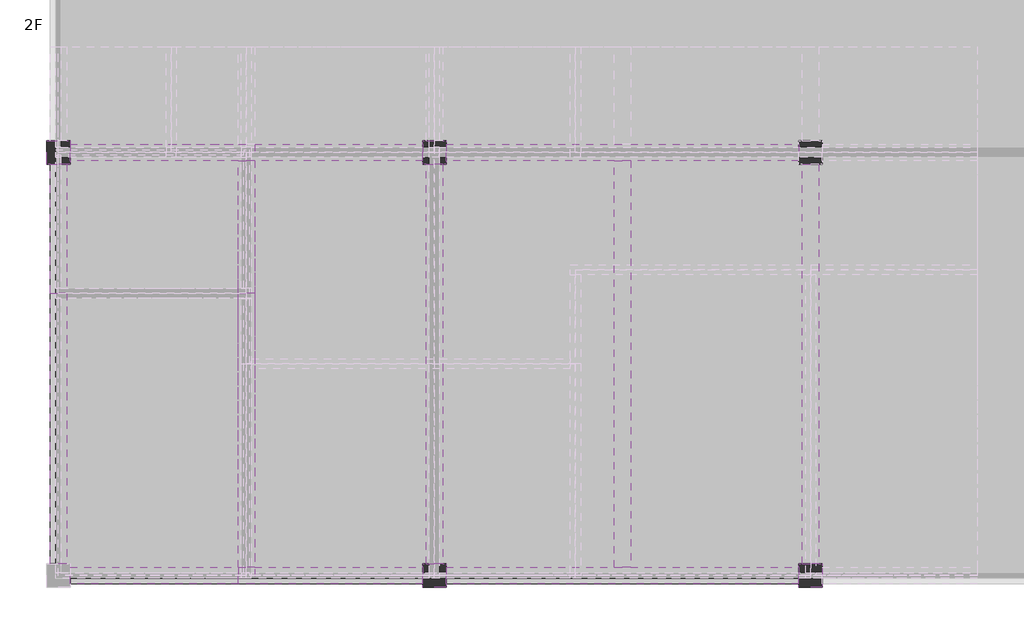
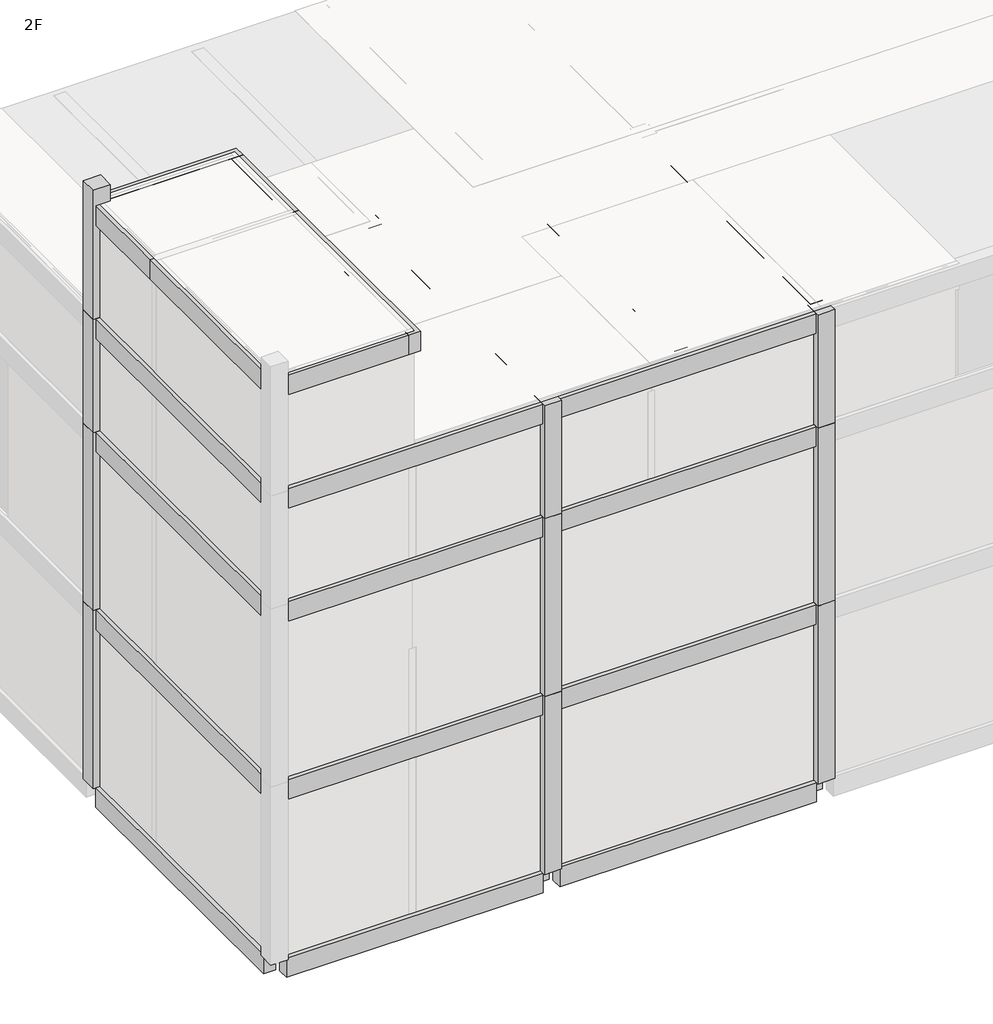
# One storey, part 4 of 7: 42 beams, 14 columns.
"""IFC4 building model written with IfcOpenShell, lengths in millimetres."""

from ifc_helpers import new_model, si_unit, frame, origin, place, context, project, spatial, polyline, outline, extrude, faceted_brep, element, save

model = new_model("IFC4")

# Units and contexts
model_context = context("Model", 3, world=origin())
ifc_project = project(units=[si_unit("LENGTHUNIT", "METRE", prefix="MILLI")], contexts=[model_context])

# Site, building, storey
site = spatial("IfcSite", under=ifc_project)
building = spatial("IfcBuilding", under=site)
storey = spatial("IfcBuildingStorey", under=building, Name="2F", Elevation=3500.0)

# Beams
placement = place(None, origin())
element("IfcBeam", 1, ObjectType="Concrete-Rectangular-Beam : BM111_400x500_RG1", at=placement, inside=storey, context=model_context, shape_type="Brep", body=[
    faceted_brep([(49634.6521483, 169923.8614395, 21500.0), (49284.6521483, 169923.8614395, 21500.0), (49284.6521483, 164098.8614395, 21500.0), (49284.6521483, 163748.8614395, 21500.0), (49634.6521483, 163748.8614395, 21500.0), (49634.6521483, 169923.8614395, 20900.0), (49634.6521483, 163748.8614395, 20900.0), (49284.6521483, 169923.8614395, 20900.0), (49284.6521483, 163748.8614395, 20900.0), (49284.6521483, 164098.8614395, 20900.0)], [[[0, 1, 2, 3, 4]], [[5, 0, 4, 6]], [[7, 5, 6, 8, 9]], [[1, 7, 9, 8, 3, 2]], [[4, 3, 8, 6]], [[1, 0, 5, 7]]]),
])
element("IfcBeam", 2, ObjectType="Concrete-Rectangular-Beam : BM111_400x500_RG1", at=placement, inside=storey, context=model_context, shape_type="SweptSolid", body=[
    extrude(outline(polyline([(49284.6521483, 164098.8614395), (49284.6521483, 163748.8614395), (45709.6521483, 163748.8614395), (45709.6521483, 164098.8614395), (49284.6521483, 164098.8614395)])), frame((0.0, 0.0, 20900.0), z_axis=(0.0, 0.0, 1.0), x_axis=(1.0, 0.0, 0.0)), (0.0, 0.0, 1.0), 600.0),
])
element("IfcBeam", 3, ObjectType="Concrete-Rectangular-Beam : BM111_400x500_RG1", at=placement, inside=storey, context=model_context, shape_type="SweptSolid", body=[
    extrude(outline(polyline([(45284.6521483, 169923.8614395), (45634.6521483, 169923.8614395), (45634.6521483, 164173.8614395), (45284.6521483, 164173.8614395), (45284.6521483, 169923.8614395)])), frame((0.0, 0.0, 20900.0), z_axis=(0.0, 0.0, 1.0), x_axis=(1.0, 0.0, 0.0)), (0.0, 0.0, 1.0), 600.0),
])
element("IfcBeam", 4, ObjectType="Concrete-Rectangular-Beam : BM111_400x500_RG1", at=placement, inside=storey, context=model_context, shape_type="Brep", body=[
    faceted_brep([(49634.6521483, 172748.8614395, 21500.0), (49634.6521483, 173098.8614395, 21500.0), (45709.6521483, 173098.8614395, 21500.0), (45709.6521483, 172748.8614395, 21500.0), (49284.6521483, 172748.8614395, 21500.0), (49634.6521483, 173098.8614395, 20900.0), (45709.6521483, 173098.8614395, 20900.0), (49634.6521483, 172748.8614395, 20900.0), (49284.6521483, 172748.8614395, 20900.0), (45709.6521483, 172748.8614395, 20900.0)], [[[0, 1, 2, 3, 4]], [[1, 5, 6, 2]], [[5, 7, 8, 9, 6]], [[7, 0, 4, 3, 9, 8]], [[1, 0, 7, 5]], [[3, 2, 6, 9]]]),
])
element("IfcBeam", 5, ObjectType="Concrete-Rectangular-Beam : BM111_400x500_RG1", at=placement, inside=storey, context=model_context, shape_type="SweptSolid", body=[
    extrude(outline(polyline([(49634.6521483, 169923.8614395), (49284.6521483, 169923.8614395), (49284.6521483, 172748.8614395), (49634.6521483, 172748.8614395), (49634.6521483, 169923.8614395)])), frame((0.0, 0.0, 20900.0), z_axis=(0.0, 0.0, 1.0), x_axis=(1.0, 0.0, 0.0)), (0.0, 0.0, 1.0), 600.0),
])
element("IfcBeam", 6, ObjectType="Concrete-Rectangular-Beam : BM111_400x500_RG1", at=placement, inside=storey, context=model_context, shape_type="SweptSolid", body=[
    extrude(outline(polyline([(45634.6521483, 169923.8614395), (45284.6521483, 169923.8614395), (45284.6521483, 172673.8614395), (45634.6521483, 172673.8614395), (45634.6521483, 169923.8614395)])), frame((0.0, 0.0, 20900.0), z_axis=(0.0, 0.0, 1.0), x_axis=(1.0, 0.0, 0.0)), (0.0, 0.0, 1.0), 600.0),
])
element("IfcBeam", 7, ObjectType="Concrete-Rectangular-Beam : BM111_400x500_RG1", at=placement, inside=storey, context=model_context, shape_type="SweptSolid", body=[
    extrude(outline(polyline([(49284.6521483, 172748.8614395), (49634.6521483, 172748.8614395), (49634.6521483, 164098.8614395), (49284.6521483, 164098.8614395), (49284.6521483, 172748.8614395)])), frame((0.0, 0.0, 2900.0), z_axis=(0.0, 0.0, 1.0), x_axis=(1.0, 0.0, 0.0)), (0.0, 0.0, 1.0), 600.0),
])
element("IfcBeam", 8, ObjectType="Concrete-Rectangular-Beam : BM111_400x500_RG1", at=placement, inside=storey, context=model_context, shape_type="SweptSolid", body=[
    extrude(outline(polyline([(57284.6521483, 172748.8614395), (57634.6521483, 172748.8614395), (57634.6521483, 164098.8614395), (57284.6521483, 164098.8614395), (57284.6521483, 172748.8614395)])), frame((0.0, 0.0, 2900.0), z_axis=(0.0, 0.0, 1.0), x_axis=(1.0, 0.0, 0.0)), (0.0, 0.0, 1.0), 600.0),
])
element("IfcBeam", 9, ObjectType="Concrete-Rectangular-Beam : BM111_400x500_RG1", at=placement, inside=storey, context=model_context, shape_type="SweptSolid", body=[
    extrude(outline(polyline([(49284.6521483, 172748.8614395), (49634.6521483, 172748.8614395), (49634.6521483, 164098.8614395), (49284.6521483, 164098.8614395), (49284.6521483, 172748.8614395)])), frame((0.0, 0.0, 8400.0), z_axis=(0.0, 0.0, 1.0), x_axis=(1.0, 0.0, 0.0)), (0.0, 0.0, 1.0), 600.0),
])
element("IfcBeam", 10, ObjectType="Concrete-Rectangular-Beam : BM111_400x500_RG1", at=placement, inside=storey, context=model_context, shape_type="SweptSolid", body=[
    extrude(outline(polyline([(57284.6521483, 172748.8614395), (57634.6521483, 172748.8614395), (57634.6521483, 164098.8614395), (57284.6521483, 164098.8614395), (57284.6521483, 172748.8614395)])), frame((0.0, 0.0, 8400.0), z_axis=(0.0, 0.0, 1.0), x_axis=(1.0, 0.0, 0.0)), (0.0, 0.0, 1.0), 600.0),
])
element("IfcBeam", 11, ObjectType="Concrete-Rectangular-Beam : BM111_400x500_RG1", at=placement, inside=storey, context=model_context, shape_type="SweptSolid", body=[
    extrude(outline(polyline([(49284.6521483, 172748.8614395), (49634.6521483, 172748.8614395), (49634.6521483, 164098.8614395), (49284.6521483, 164098.8614395), (49284.6521483, 172748.8614395)])), frame((0.0, 0.0, 13900.0), z_axis=(0.0, 0.0, 1.0), x_axis=(1.0, 0.0, 0.0)), (0.0, 0.0, 1.0), 600.0),
])
element("IfcBeam", 12, ObjectType="Concrete-Rectangular-Beam : BM111_400x500_RG1", at=placement, inside=storey, context=model_context, shape_type="SweptSolid", body=[
    extrude(outline(polyline([(57284.6521483, 172748.8614395), (57634.6521483, 172748.8614395), (57634.6521483, 164098.8614395), (57284.6521483, 164098.8614395), (57284.6521483, 172748.8614395)])), frame((0.0, 0.0, 13900.0), z_axis=(0.0, 0.0, 1.0), x_axis=(1.0, 0.0, 0.0)), (0.0, 0.0, 1.0), 600.0),
])
element("IfcBeam", 13, ObjectType="Concrete-Rectangular-Beam : BM111_400x500_RG1", at=placement, inside=storey, context=model_context, shape_type="SweptSolid", body=[
    extrude(outline(polyline([(49284.6521483, 172748.8614395), (49634.6521483, 172748.8614395), (49634.6521483, 164098.8614395), (49284.6521483, 164098.8614395), (49284.6521483, 172748.8614395)])), frame((0.0, 0.0, 17400.0), z_axis=(0.0, 0.0, 1.0), x_axis=(1.0, 0.0, 0.0)), (0.0, 0.0, 1.0), 600.0),
])
element("IfcBeam", 14, ObjectType="Concrete-Rectangular-Beam : BM111_400x500_RG1", at=placement, inside=storey, context=model_context, shape_type="SweptSolid", body=[
    extrude(outline(polyline([(57284.6521483, 172748.8614395), (57634.6521483, 172748.8614395), (57634.6521483, 164098.8614395), (57284.6521483, 164098.8614395), (57284.6521483, 172748.8614395)])), frame((0.0, 0.0, 17400.0), z_axis=(0.0, 0.0, 1.0), x_axis=(1.0, 0.0, 0.0)), (0.0, 0.0, 1.0), 600.0),
])
element("IfcBeam", 15, ObjectType="Concrete-Rectangular-Beam : BM111_400x500_RG1", at=placement, inside=storey, context=model_context, shape_type="Brep", body=[
    faceted_brep([(45709.6521483, 173098.8614395, 3500.0), (45709.6521483, 172748.8614395, 3500.0), (49284.6521483, 172748.8614395, 3500.0), (49634.6521483, 172748.8614395, 3500.0), (53209.6521483, 172748.8614395, 3500.0), (53209.6521483, 173098.8614395, 3500.0), (49634.6521483, 173098.8614395, 3500.0), (49284.6521483, 173098.8614395, 3500.0), (45709.6521483, 172748.8614395, 2900.0), (49284.6521483, 172748.8614395, 2900.0), (49634.6521483, 172748.8614395, 2900.0), (53209.6521483, 172748.8614395, 2900.0), (45709.6521483, 173098.8614395, 2900.0), (49284.6521483, 173098.8614395, 2900.0), (49634.6521483, 173098.8614395, 2900.0), (53209.6521483, 173098.8614395, 2900.0)], [[[0, 1, 2, 3, 4, 5, 6, 7]], [[1, 8, 9, 10, 11, 4, 3, 2]], [[8, 12, 13, 14, 15, 11, 10, 9]], [[12, 0, 7, 6, 5, 15, 14, 13]], [[1, 0, 12, 8]], [[5, 4, 11, 15]]]),
])
element("IfcBeam", 16, ObjectType="Concrete-Rectangular-Beam : BM111_400x500_RG1", at=placement, inside=storey, context=model_context, shape_type="Brep", body=[
    faceted_brep([(53709.6521483, 173098.8614395, 3500.0), (53709.6521483, 172748.8614395, 3500.0), (57284.6521483, 172748.8614395, 3500.0), (57634.6521483, 172748.8614395, 3500.0), (61209.6521483, 172748.8614395, 3500.0), (61209.6521483, 173098.8614395, 3500.0), (57634.6521483, 173098.8614395, 3500.0), (57284.6521483, 173098.8614395, 3500.0), (53709.6521483, 172748.8614395, 2900.0), (57284.6521483, 172748.8614395, 2900.0), (57634.6521483, 172748.8614395, 2900.0), (61209.6521483, 172748.8614395, 2900.0), (53709.6521483, 173098.8614395, 2900.0), (57284.6521483, 173098.8614395, 2900.0), (57634.6521483, 173098.8614395, 2900.0), (61209.6521483, 173098.8614395, 2900.0)], [[[0, 1, 2, 3, 4, 5, 6, 7]], [[1, 8, 9, 10, 11, 4, 3, 2]], [[8, 12, 13, 14, 15, 11, 10, 9]], [[12, 0, 7, 6, 5, 15, 14, 13]], [[1, 0, 12, 8]], [[5, 4, 11, 15]]]),
])
element("IfcBeam", 17, ObjectType="Concrete-Rectangular-Beam : BM111_400x500_RG1", at=placement, inside=storey, context=model_context, shape_type="Brep", body=[
    faceted_brep([(45709.6521483, 164098.8614395, 3500.0), (45709.6521483, 163748.8614395, 3500.0), (53209.6521483, 163748.8614395, 3500.0), (53209.6521483, 164098.8614395, 3500.0), (49634.6521483, 164098.8614395, 3500.0), (49284.6521483, 164098.8614395, 3500.0), (45709.6521483, 163748.8614395, 2900.0), (53209.6521483, 163748.8614395, 2900.0), (45709.6521483, 164098.8614395, 2900.0), (49284.6521483, 164098.8614395, 2900.0), (49634.6521483, 164098.8614395, 2900.0), (53209.6521483, 164098.8614395, 2900.0)], [[[0, 1, 2, 3, 4, 5]], [[1, 6, 7, 2]], [[6, 8, 9, 10, 11, 7]], [[8, 0, 5, 4, 3, 11, 10, 9]], [[1, 0, 8, 6]], [[3, 2, 7, 11]]]),
])
element("IfcBeam", 18, ObjectType="Concrete-Rectangular-Beam : BM111_400x500_RG1", at=placement, inside=storey, context=model_context, shape_type="Brep", body=[
    faceted_brep([(53709.6521483, 164098.8614395, 3500.0), (53709.6521483, 163748.8614395, 3500.0), (61209.6521483, 163748.8614395, 3500.0), (61209.6521483, 164098.8614395, 3500.0), (57634.6521483, 164098.8614395, 3500.0), (57284.6521483, 164098.8614395, 3500.0), (53709.6521483, 163748.8614395, 2900.0), (61209.6521483, 163748.8614395, 2900.0), (53709.6521483, 164098.8614395, 2900.0), (57284.6521483, 164098.8614395, 2900.0), (57634.6521483, 164098.8614395, 2900.0), (61209.6521483, 164098.8614395, 2900.0)], [[[0, 1, 2, 3, 4, 5]], [[1, 6, 7, 2]], [[6, 8, 9, 10, 11, 7]], [[8, 0, 5, 4, 3, 11, 10, 9]], [[1, 0, 8, 6]], [[3, 2, 7, 11]]]),
])
element("IfcBeam", 19, ObjectType="Concrete-Rectangular-Beam : BM111_400x500_RG1", at=placement, inside=storey, context=model_context, shape_type="Brep", body=[
    faceted_brep([(45709.6521483, 173098.8614395, 9000.0), (45709.6521483, 172748.8614395, 9000.0), (49284.6521483, 172748.8614395, 9000.0), (49634.6521483, 172748.8614395, 9000.0), (53209.6521483, 172748.8614395, 9000.0), (53209.6521483, 173098.8614395, 9000.0), (49634.6521483, 173098.8614395, 9000.0), (49284.6521483, 173098.8614395, 9000.0), (45709.6521483, 172748.8614395, 8400.0), (49284.6521483, 172748.8614395, 8400.0), (49634.6521483, 172748.8614395, 8400.0), (53209.6521483, 172748.8614395, 8400.0), (45709.6521483, 173098.8614395, 8400.0), (49284.6521483, 173098.8614395, 8400.0), (49634.6521483, 173098.8614395, 8400.0), (53209.6521483, 173098.8614395, 8400.0)], [[[0, 1, 2, 3, 4, 5, 6, 7]], [[1, 8, 9, 10, 11, 4, 3, 2]], [[8, 12, 13, 14, 15, 11, 10, 9]], [[12, 0, 7, 6, 5, 15, 14, 13]], [[1, 0, 12, 8]], [[5, 4, 11, 15]]]),
])
element("IfcBeam", 20, ObjectType="Concrete-Rectangular-Beam : BM111_400x500_RG1", at=placement, inside=storey, context=model_context, shape_type="Brep", body=[
    faceted_brep([(53709.6521483, 173098.8614395, 9000.0), (53709.6521483, 172748.8614395, 9000.0), (57284.6521483, 172748.8614395, 9000.0), (57634.6521483, 172748.8614395, 9000.0), (61209.6521483, 172748.8614395, 9000.0), (61209.6521483, 173098.8614395, 9000.0), (57634.6521483, 173098.8614395, 9000.0), (57284.6521483, 173098.8614395, 9000.0), (53709.6521483, 172748.8614395, 8400.0), (57284.6521483, 172748.8614395, 8400.0), (57634.6521483, 172748.8614395, 8400.0), (61209.6521483, 172748.8614395, 8400.0), (53709.6521483, 173098.8614395, 8400.0), (57284.6521483, 173098.8614395, 8400.0), (57634.6521483, 173098.8614395, 8400.0), (61209.6521483, 173098.8614395, 8400.0)], [[[0, 1, 2, 3, 4, 5, 6, 7]], [[1, 8, 9, 10, 11, 4, 3, 2]], [[8, 12, 13, 14, 15, 11, 10, 9]], [[12, 0, 7, 6, 5, 15, 14, 13]], [[1, 0, 12, 8]], [[5, 4, 11, 15]]]),
])
element("IfcBeam", 21, ObjectType="Concrete-Rectangular-Beam : BM111_400x500_RG1", at=placement, inside=storey, context=model_context, shape_type="Brep", body=[
    faceted_brep([(45709.6521483, 164098.8614395, 9000.0), (45709.6521483, 163748.8614395, 9000.0), (53209.6521483, 163748.8614395, 9000.0), (53209.6521483, 164098.8614395, 9000.0), (49634.6521483, 164098.8614395, 9000.0), (49284.6521483, 164098.8614395, 9000.0), (45709.6521483, 163748.8614395, 8400.0), (53209.6521483, 163748.8614395, 8400.0), (45709.6521483, 164098.8614395, 8400.0), (49284.6521483, 164098.8614395, 8400.0), (49634.6521483, 164098.8614395, 8400.0), (53209.6521483, 164098.8614395, 8400.0)], [[[0, 1, 2, 3, 4, 5]], [[1, 6, 7, 2]], [[6, 8, 9, 10, 11, 7]], [[8, 0, 5, 4, 3, 11, 10, 9]], [[1, 0, 8, 6]], [[3, 2, 7, 11]]]),
])
element("IfcBeam", 22, ObjectType="Concrete-Rectangular-Beam : BM111_400x500_RG1", at=placement, inside=storey, context=model_context, shape_type="Brep", body=[
    faceted_brep([(53709.6521483, 164098.8614395, 9000.0), (53709.6521483, 163748.8614395, 9000.0), (61209.6521483, 163748.8614395, 9000.0), (61209.6521483, 164098.8614395, 9000.0), (57634.6521483, 164098.8614395, 9000.0), (57284.6521483, 164098.8614395, 9000.0), (53709.6521483, 163748.8614395, 8400.0), (61209.6521483, 163748.8614395, 8400.0), (53709.6521483, 164098.8614395, 8400.0), (57284.6521483, 164098.8614395, 8400.0), (57634.6521483, 164098.8614395, 8400.0), (61209.6521483, 164098.8614395, 8400.0)], [[[0, 1, 2, 3, 4, 5]], [[1, 6, 7, 2]], [[6, 8, 9, 10, 11, 7]], [[8, 0, 5, 4, 3, 11, 10, 9]], [[1, 0, 8, 6]], [[3, 2, 7, 11]]]),
])
element("IfcBeam", 23, ObjectType="Concrete-Rectangular-Beam : BM111_400x500_RG1", at=placement, inside=storey, context=model_context, shape_type="Brep", body=[
    faceted_brep([(45709.6521483, 173098.8614395, 14500.0), (45709.6521483, 172748.8614395, 14500.0), (49284.6521483, 172748.8614395, 14500.0), (49634.6521483, 172748.8614395, 14500.0), (53209.6521483, 172748.8614395, 14500.0), (53209.6521483, 173098.8614395, 14500.0), (49634.6521483, 173098.8614395, 14500.0), (49284.6521483, 173098.8614395, 14500.0), (45709.6521483, 172748.8614395, 13900.0), (49284.6521483, 172748.8614395, 13900.0), (49634.6521483, 172748.8614395, 13900.0), (53209.6521483, 172748.8614395, 13900.0), (45709.6521483, 173098.8614395, 13900.0), (49284.6521483, 173098.8614395, 13900.0), (49634.6521483, 173098.8614395, 13900.0), (53209.6521483, 173098.8614395, 13900.0)], [[[0, 1, 2, 3, 4, 5, 6, 7]], [[1, 8, 9, 10, 11, 4, 3, 2]], [[8, 12, 13, 14, 15, 11, 10, 9]], [[12, 0, 7, 6, 5, 15, 14, 13]], [[1, 0, 12, 8]], [[5, 4, 11, 15]]]),
])
element("IfcBeam", 24, ObjectType="Concrete-Rectangular-Beam : BM111_400x500_RG1", at=placement, inside=storey, context=model_context, shape_type="Brep", body=[
    faceted_brep([(53709.6521483, 173098.8614395, 14500.0), (53709.6521483, 172748.8614395, 14500.0), (57284.6521483, 172748.8614395, 14500.0), (57634.6521483, 172748.8614395, 14500.0), (61209.6521483, 172748.8614395, 14500.0), (61209.6521483, 173098.8614395, 14500.0), (57634.6521483, 173098.8614395, 14500.0), (57284.6521483, 173098.8614395, 14500.0), (53709.6521483, 172748.8614395, 13900.0), (57284.6521483, 172748.8614395, 13900.0), (57634.6521483, 172748.8614395, 13900.0), (61209.6521483, 172748.8614395, 13900.0), (53709.6521483, 173098.8614395, 13900.0), (57284.6521483, 173098.8614395, 13900.0), (57634.6521483, 173098.8614395, 13900.0), (61209.6521483, 173098.8614395, 13900.0)], [[[0, 1, 2, 3, 4, 5, 6, 7]], [[1, 8, 9, 10, 11, 4, 3, 2]], [[8, 12, 13, 14, 15, 11, 10, 9]], [[12, 0, 7, 6, 5, 15, 14, 13]], [[1, 0, 12, 8]], [[5, 4, 11, 15]]]),
])
element("IfcBeam", 25, ObjectType="Concrete-Rectangular-Beam : BM111_400x500_RG1", at=placement, inside=storey, context=model_context, shape_type="Brep", body=[
    faceted_brep([(45709.6521483, 164098.8614395, 14500.0), (45709.6521483, 163748.8614395, 14500.0), (53209.6521483, 163748.8614395, 14500.0), (53209.6521483, 164098.8614395, 14500.0), (49634.6521483, 164098.8614395, 14500.0), (49284.6521483, 164098.8614395, 14500.0), (45709.6521483, 163748.8614395, 13900.0), (53209.6521483, 163748.8614395, 13900.0), (45709.6521483, 164098.8614395, 13900.0), (49284.6521483, 164098.8614395, 13900.0), (49634.6521483, 164098.8614395, 13900.0), (53209.6521483, 164098.8614395, 13900.0)], [[[0, 1, 2, 3, 4, 5]], [[1, 6, 7, 2]], [[6, 8, 9, 10, 11, 7]], [[8, 0, 5, 4, 3, 11, 10, 9]], [[1, 0, 8, 6]], [[3, 2, 7, 11]]]),
])
element("IfcBeam", 26, ObjectType="Concrete-Rectangular-Beam : BM111_400x500_RG1", at=placement, inside=storey, context=model_context, shape_type="Brep", body=[
    faceted_brep([(53709.6521483, 164098.8614395, 14500.0), (53709.6521483, 163748.8614395, 14500.0), (61209.6521483, 163748.8614395, 14500.0), (61209.6521483, 164098.8614395, 14500.0), (57634.6521483, 164098.8614395, 14500.0), (57284.6521483, 164098.8614395, 14500.0), (53709.6521483, 163748.8614395, 13900.0), (61209.6521483, 163748.8614395, 13900.0), (53709.6521483, 164098.8614395, 13900.0), (57284.6521483, 164098.8614395, 13900.0), (57634.6521483, 164098.8614395, 13900.0), (61209.6521483, 164098.8614395, 13900.0)], [[[0, 1, 2, 3, 4, 5]], [[1, 6, 7, 2]], [[6, 8, 9, 10, 11, 7]], [[8, 0, 5, 4, 3, 11, 10, 9]], [[1, 0, 8, 6]], [[3, 2, 7, 11]]]),
])
element("IfcBeam", 27, ObjectType="Concrete-Rectangular-Beam : BM111_400x500_RG1", at=placement, inside=storey, context=model_context, shape_type="Brep", body=[
    faceted_brep([(45709.6521483, 173098.8614395, 18000.0), (45709.6521483, 172748.8614395, 18000.0), (49284.6521483, 172748.8614395, 18000.0), (49634.6521483, 172748.8614395, 18000.0), (53209.6521483, 172748.8614395, 18000.0), (53209.6521483, 173098.8614395, 18000.0), (49634.6521483, 173098.8614395, 18000.0), (49284.6521483, 173098.8614395, 18000.0), (45709.6521483, 172748.8614395, 17400.0), (49284.6521483, 172748.8614395, 17400.0), (49634.6521483, 172748.8614395, 17400.0), (53209.6521483, 172748.8614395, 17400.0), (45709.6521483, 173098.8614395, 17400.0), (49284.6521483, 173098.8614395, 17400.0), (49634.6521483, 173098.8614395, 17400.0), (53209.6521483, 173098.8614395, 17400.0)], [[[0, 1, 2, 3, 4, 5, 6, 7]], [[1, 8, 9, 10, 11, 4, 3, 2]], [[8, 12, 13, 14, 15, 11, 10, 9]], [[12, 0, 7, 6, 5, 15, 14, 13]], [[1, 0, 12, 8]], [[5, 4, 11, 15]]]),
])
element("IfcBeam", 28, ObjectType="Concrete-Rectangular-Beam : BM111_400x500_RG1", at=placement, inside=storey, context=model_context, shape_type="Brep", body=[
    faceted_brep([(53709.6521483, 173098.8614395, 18000.0), (53709.6521483, 172748.8614395, 18000.0), (57284.6521483, 172748.8614395, 18000.0), (57634.6521483, 172748.8614395, 18000.0), (61209.6521483, 172748.8614395, 18000.0), (61209.6521483, 173098.8614395, 18000.0), (57634.6521483, 173098.8614395, 18000.0), (57284.6521483, 173098.8614395, 18000.0), (53709.6521483, 172748.8614395, 17400.0), (57284.6521483, 172748.8614395, 17400.0), (57634.6521483, 172748.8614395, 17400.0), (61209.6521483, 172748.8614395, 17400.0), (53709.6521483, 173098.8614395, 17400.0), (57284.6521483, 173098.8614395, 17400.0), (57634.6521483, 173098.8614395, 17400.0), (61209.6521483, 173098.8614395, 17400.0)], [[[0, 1, 2, 3, 4, 5, 6, 7]], [[1, 8, 9, 10, 11, 4, 3, 2]], [[8, 12, 13, 14, 15, 11, 10, 9]], [[12, 0, 7, 6, 5, 15, 14, 13]], [[1, 0, 12, 8]], [[5, 4, 11, 15]]]),
])
element("IfcBeam", 29, ObjectType="Concrete-Rectangular-Beam : BM111_400x500_RG1", at=placement, inside=storey, context=model_context, shape_type="Brep", body=[
    faceted_brep([(45709.6521483, 164098.8614395, 18000.0), (45709.6521483, 163748.8614395, 18000.0), (53209.6521483, 163748.8614395, 18000.0), (53209.6521483, 164098.8614395, 18000.0), (49634.6521483, 164098.8614395, 18000.0), (49284.6521483, 164098.8614395, 18000.0), (45709.6521483, 163748.8614395, 17400.0), (53209.6521483, 163748.8614395, 17400.0), (45709.6521483, 164098.8614395, 17400.0), (49284.6521483, 164098.8614395, 17400.0), (49634.6521483, 164098.8614395, 17400.0), (53209.6521483, 164098.8614395, 17400.0)], [[[0, 1, 2, 3, 4, 5]], [[1, 6, 7, 2]], [[6, 8, 9, 10, 11, 7]], [[8, 0, 5, 4, 3, 11, 10, 9]], [[1, 0, 8, 6]], [[3, 2, 7, 11]]]),
])
element("IfcBeam", 30, ObjectType="Concrete-Rectangular-Beam : BM111_400x500_RG1", at=placement, inside=storey, context=model_context, shape_type="Brep", body=[
    faceted_brep([(53709.6521483, 164098.8614395, 18000.0), (53709.6521483, 163748.8614395, 18000.0), (61209.6521483, 163748.8614395, 18000.0), (61209.6521483, 164098.8614395, 18000.0), (57634.6521483, 164098.8614395, 18000.0), (57284.6521483, 164098.8614395, 18000.0), (53709.6521483, 163748.8614395, 17400.0), (61209.6521483, 163748.8614395, 17400.0), (53709.6521483, 164098.8614395, 17400.0), (57284.6521483, 164098.8614395, 17400.0), (57634.6521483, 164098.8614395, 17400.0), (61209.6521483, 164098.8614395, 17400.0)], [[[0, 1, 2, 3, 4, 5]], [[1, 6, 7, 2]], [[6, 8, 9, 10, 11, 7]], [[8, 0, 5, 4, 3, 11, 10, 9]], [[1, 0, 8, 6]], [[3, 2, 7, 11]]]),
])
element("IfcBeam", 31, ObjectType="Concrete-Rectangular-Beam : BM111_400x500_RG1", at=placement, inside=storey, context=model_context, shape_type="SweptSolid", body=[
    extrude(outline(polyline([(45284.6521483, 172673.8614395), (45634.6521483, 172673.8614395), (45634.6521483, 164173.8614395), (45284.6521483, 164173.8614395), (45284.6521483, 172673.8614395)])), frame((0.0, 0.0, 2900.0), z_axis=(0.0, 0.0, 1.0), x_axis=(1.0, 0.0, 0.0)), (0.0, 0.0, 1.0), 600.0),
])
element("IfcBeam", 32, ObjectType="Concrete-Rectangular-Beam : BM111_400x500_RG1", at=placement, inside=storey, context=model_context, shape_type="SweptSolid", body=[
    extrude(outline(polyline([(53284.6521483, 172673.8614395), (53634.6521483, 172673.8614395), (53634.6521483, 164173.8614395), (53284.6521483, 164173.8614395), (53284.6521483, 172673.8614395)])), frame((0.0, 0.0, 2900.0), z_axis=(0.0, 0.0, 1.0), x_axis=(1.0, 0.0, 0.0)), (0.0, 0.0, 1.0), 600.0),
])
element("IfcBeam", 33, ObjectType="Concrete-Rectangular-Beam : BM111_400x500_RG1", at=placement, inside=storey, context=model_context, shape_type="SweptSolid", body=[
    extrude(outline(polyline([(61284.6521483, 172673.8614395), (61634.6521483, 172673.8614395), (61634.6521483, 164173.8614395), (61284.6521483, 164173.8614395), (61284.6521483, 172673.8614395)])), frame((0.0, 0.0, 2900.0), z_axis=(0.0, 0.0, 1.0), x_axis=(1.0, 0.0, 0.0)), (0.0, 0.0, 1.0), 600.0),
])
element("IfcBeam", 34, ObjectType="Concrete-Rectangular-Beam : BM111_400x500_RG1", at=placement, inside=storey, context=model_context, shape_type="SweptSolid", body=[
    extrude(outline(polyline([(45284.6521483, 172673.8614395), (45634.6521483, 172673.8614395), (45634.6521483, 164173.8614395), (45284.6521483, 164173.8614395), (45284.6521483, 172673.8614395)])), frame((0.0, 0.0, 8400.0), z_axis=(0.0, 0.0, 1.0), x_axis=(1.0, 0.0, 0.0)), (0.0, 0.0, 1.0), 600.0),
])
element("IfcBeam", 35, ObjectType="Concrete-Rectangular-Beam : BM111_400x500_RG1", at=placement, inside=storey, context=model_context, shape_type="SweptSolid", body=[
    extrude(outline(polyline([(53284.6521483, 172673.8614395), (53634.6521483, 172673.8614395), (53634.6521483, 164173.8614395), (53284.6521483, 164173.8614395), (53284.6521483, 172673.8614395)])), frame((0.0, 0.0, 8400.0), z_axis=(0.0, 0.0, 1.0), x_axis=(1.0, 0.0, 0.0)), (0.0, 0.0, 1.0), 600.0),
])
element("IfcBeam", 36, ObjectType="Concrete-Rectangular-Beam : BM111_400x500_RG1", at=placement, inside=storey, context=model_context, shape_type="SweptSolid", body=[
    extrude(outline(polyline([(61284.6521483, 172673.8614395), (61634.6521483, 172673.8614395), (61634.6521483, 164173.8614395), (61284.6521483, 164173.8614395), (61284.6521483, 172673.8614395)])), frame((0.0, 0.0, 8400.0), z_axis=(0.0, 0.0, 1.0), x_axis=(1.0, 0.0, 0.0)), (0.0, 0.0, 1.0), 600.0),
])
element("IfcBeam", 37, ObjectType="Concrete-Rectangular-Beam : BM111_400x500_RG1", at=placement, inside=storey, context=model_context, shape_type="SweptSolid", body=[
    extrude(outline(polyline([(45284.6521483, 172673.8614395), (45634.6521483, 172673.8614395), (45634.6521483, 164173.8614395), (45284.6521483, 164173.8614395), (45284.6521483, 172673.8614395)])), frame((0.0, 0.0, 13900.0), z_axis=(0.0, 0.0, 1.0), x_axis=(1.0, 0.0, 0.0)), (0.0, 0.0, 1.0), 600.0),
])
element("IfcBeam", 38, ObjectType="Concrete-Rectangular-Beam : BM111_400x500_RG1", at=placement, inside=storey, context=model_context, shape_type="SweptSolid", body=[
    extrude(outline(polyline([(53284.6521483, 172673.8614395), (53634.6521483, 172673.8614395), (53634.6521483, 164173.8614395), (53284.6521483, 164173.8614395), (53284.6521483, 172673.8614395)])), frame((0.0, 0.0, 13900.0), z_axis=(0.0, 0.0, 1.0), x_axis=(1.0, 0.0, 0.0)), (0.0, 0.0, 1.0), 600.0),
])
element("IfcBeam", 39, ObjectType="Concrete-Rectangular-Beam : BM111_400x500_RG1", at=placement, inside=storey, context=model_context, shape_type="SweptSolid", body=[
    extrude(outline(polyline([(61284.6521483, 172673.8614395), (61634.6521483, 172673.8614395), (61634.6521483, 164173.8614395), (61284.6521483, 164173.8614395), (61284.6521483, 172673.8614395)])), frame((0.0, 0.0, 13900.0), z_axis=(0.0, 0.0, 1.0), x_axis=(1.0, 0.0, 0.0)), (0.0, 0.0, 1.0), 600.0),
])
element("IfcBeam", 40, ObjectType="Concrete-Rectangular-Beam : BM111_400x500_RG1", at=placement, inside=storey, context=model_context, shape_type="SweptSolid", body=[
    extrude(outline(polyline([(45284.6521483, 172673.8614395), (45634.6521483, 172673.8614395), (45634.6521483, 164173.8614395), (45284.6521483, 164173.8614395), (45284.6521483, 172673.8614395)])), frame((0.0, 0.0, 17400.0), z_axis=(0.0, 0.0, 1.0), x_axis=(1.0, 0.0, 0.0)), (0.0, 0.0, 1.0), 600.0),
])
element("IfcBeam", 41, ObjectType="Concrete-Rectangular-Beam : BM111_400x500_RG1", at=placement, inside=storey, context=model_context, shape_type="SweptSolid", body=[
    extrude(outline(polyline([(53284.6521483, 172673.8614395), (53634.6521483, 172673.8614395), (53634.6521483, 164173.8614395), (53284.6521483, 164173.8614395), (53284.6521483, 172673.8614395)])), frame((0.0, 0.0, 17400.0), z_axis=(0.0, 0.0, 1.0), x_axis=(1.0, 0.0, 0.0)), (0.0, 0.0, 1.0), 600.0),
])
element("IfcBeam", 42, ObjectType="Concrete-Rectangular-Beam : BM111_400x500_RG1", at=placement, inside=storey, context=model_context, shape_type="SweptSolid", body=[
    extrude(outline(polyline([(61284.6521483, 172673.8614395), (61634.6521483, 172673.8614395), (61634.6521483, 164173.8614395), (61284.6521483, 164173.8614395), (61284.6521483, 172673.8614395)])), frame((0.0, 0.0, 17400.0), z_axis=(0.0, 0.0, 1.0), x_axis=(1.0, 0.0, 0.0)), (0.0, 0.0, 1.0), 600.0),
])

# Columns
element("IfcColumn", 43, ObjectType="Concrete-Rectangular-Column : CL111_500x500", at=placement, inside=storey, context=model_context, shape_type="Brep", body=[
    faceted_brep([(45709.6521483, 173173.8614395, 3500.0), (45709.6521483, 172673.8614395, 3500.0), (45209.6521483, 172673.8614395, 3500.0), (45209.6521483, 173173.8614395, 3500.0), (45709.6521483, 173173.8614395, 9000.0), (45709.6521483, 173098.8614395, 9000.0), (45709.6521483, 172748.8614395, 9000.0), (45709.6521483, 172673.8614395, 9000.0), (45634.6521483, 172673.8614395, 9000.0), (45284.6521483, 172673.8614395, 9000.0), (45209.6521483, 172673.8614395, 9000.0), (45209.6521483, 173173.8614395, 9000.0), (45284.6521483, 173173.8614395, 9000.0), (45634.6521483, 173173.8614395, 9000.0)], [[[0, 1, 2, 3]], [[4, 5, 6, 7, 1, 0]], [[7, 8, 9, 10, 2, 1]], [[10, 11, 3, 2]], [[11, 12, 13, 4, 0, 3]], [[4, 13, 12, 11, 10, 9, 8, 7, 6, 5]]]),
])
element("IfcColumn", 44, ObjectType="Concrete-Rectangular-Column : CL111_500x500", at=placement, inside=storey, context=model_context, shape_type="Brep", body=[
    faceted_brep([(45709.6521483, 173173.8614395, 9000.0), (45709.6521483, 172673.8614395, 9000.0), (45209.6521483, 172673.8614395, 9000.0), (45209.6521483, 173173.8614395, 9000.0), (45709.6521483, 173173.8614395, 14500.0), (45709.6521483, 173098.8614395, 14500.0), (45709.6521483, 172748.8614395, 14500.0), (45709.6521483, 172673.8614395, 14500.0), (45634.6521483, 172673.8614395, 14500.0), (45284.6521483, 172673.8614395, 14500.0), (45209.6521483, 172673.8614395, 14500.0), (45209.6521483, 173173.8614395, 14500.0), (45284.6521483, 173173.8614395, 14500.0), (45634.6521483, 173173.8614395, 14500.0)], [[[0, 1, 2, 3]], [[4, 5, 6, 7, 1, 0]], [[7, 8, 9, 10, 2, 1]], [[10, 11, 3, 2]], [[11, 12, 13, 4, 0, 3]], [[4, 13, 12, 11, 10, 9, 8, 7, 6, 5]]]),
])
element("IfcColumn", 45, ObjectType="Concrete-Rectangular-Column : CL111_500x500", at=placement, inside=storey, context=model_context, shape_type="Brep", body=[
    faceted_brep([(45709.6521483, 173173.8614395, 14500.0), (45709.6521483, 172673.8614395, 14500.0), (45209.6521483, 172673.8614395, 14500.0), (45209.6521483, 173173.8614395, 14500.0), (45709.6521483, 173173.8614395, 18000.0), (45709.6521483, 173098.8614395, 18000.0), (45709.6521483, 172748.8614395, 18000.0), (45709.6521483, 172673.8614395, 18000.0), (45634.6521483, 172673.8614395, 18000.0), (45284.6521483, 172673.8614395, 18000.0), (45209.6521483, 172673.8614395, 18000.0), (45209.6521483, 173173.8614395, 18000.0), (45284.6521483, 173173.8614395, 18000.0), (45634.6521483, 173173.8614395, 18000.0)], [[[0, 1, 2, 3]], [[4, 5, 6, 7, 1, 0]], [[7, 8, 9, 10, 2, 1]], [[10, 11, 3, 2]], [[11, 12, 13, 4, 0, 3]], [[4, 13, 12, 11, 10, 9, 8, 7, 6, 5]]]),
])
element("IfcColumn", 46, ObjectType="Concrete-Rectangular-Column : CL111_500x500", at=placement, inside=storey, context=model_context, shape_type="SweptSolid", body=[
    extrude(outline(polyline([(45709.6521483, 173173.8614395), (45709.6521483, 172673.8614395), (45209.6521483, 172673.8614395), (45209.6521483, 173173.8614395), (45709.6521483, 173173.8614395)])), frame((0.0, 0.0, 18000.0), z_axis=(0.0, 0.0, 1.0), x_axis=(1.0, 0.0, 0.0)), (0.0, 0.0, 1.0), 4000.0),
])
element("IfcColumn", 47, ObjectType="Concrete-Rectangular-Column : CL111_500x500", at=placement, inside=storey, context=model_context, shape_type="Brep", body=[
    faceted_brep([(53709.6521483, 173173.8614395, 3500.0), (53709.6521483, 172673.8614395, 3500.0), (53209.6521483, 172673.8614395, 3500.0), (53209.6521483, 173173.8614395, 3500.0), (53709.6521483, 173173.8614395, 9000.0), (53709.6521483, 173098.8614395, 9000.0), (53709.6521483, 172748.8614395, 9000.0), (53709.6521483, 172673.8614395, 9000.0), (53634.6521483, 172673.8614395, 9000.0), (53284.6521483, 172673.8614395, 9000.0), (53209.6521483, 172673.8614395, 9000.0), (53209.6521483, 172748.8614395, 9000.0), (53209.6521483, 173098.8614395, 9000.0), (53209.6521483, 173173.8614395, 9000.0), (53284.6521483, 173173.8614395, 9000.0), (53634.6521483, 173173.8614395, 9000.0)], [[[0, 1, 2, 3]], [[4, 5, 6, 7, 1, 0]], [[7, 8, 9, 10, 2, 1]], [[10, 11, 12, 13, 3, 2]], [[13, 14, 15, 4, 0, 3]], [[4, 15, 14, 13, 12, 11, 10, 9, 8, 7, 6, 5]]]),
])
element("IfcColumn", 48, ObjectType="Concrete-Rectangular-Column : CL111_500x500", at=placement, inside=storey, context=model_context, shape_type="Brep", body=[
    faceted_brep([(53709.6521483, 173173.8614395, 9000.0), (53709.6521483, 172673.8614395, 9000.0), (53209.6521483, 172673.8614395, 9000.0), (53209.6521483, 173173.8614395, 9000.0), (53709.6521483, 173173.8614395, 14500.0), (53709.6521483, 173098.8614395, 14500.0), (53709.6521483, 172748.8614395, 14500.0), (53709.6521483, 172673.8614395, 14500.0), (53634.6521483, 172673.8614395, 14500.0), (53284.6521483, 172673.8614395, 14500.0), (53209.6521483, 172673.8614395, 14500.0), (53209.6521483, 172748.8614395, 14500.0), (53209.6521483, 173098.8614395, 14500.0), (53209.6521483, 173173.8614395, 14500.0), (53284.6521483, 173173.8614395, 14500.0), (53634.6521483, 173173.8614395, 14500.0)], [[[0, 1, 2, 3]], [[4, 5, 6, 7, 1, 0]], [[7, 8, 9, 10, 2, 1]], [[10, 11, 12, 13, 3, 2]], [[13, 14, 15, 4, 0, 3]], [[4, 15, 14, 13, 12, 11, 10, 9, 8, 7, 6, 5]]]),
])
element("IfcColumn", 49, ObjectType="Concrete-Rectangular-Column : CL111_500x500", at=placement, inside=storey, context=model_context, shape_type="Brep", body=[
    faceted_brep([(53709.6521483, 173173.8614395, 14500.0), (53709.6521483, 172673.8614395, 14500.0), (53209.6521483, 172673.8614395, 14500.0), (53209.6521483, 173173.8614395, 14500.0), (53709.6521483, 173173.8614395, 18000.0), (53709.6521483, 173098.8614395, 18000.0), (53709.6521483, 172748.8614395, 18000.0), (53709.6521483, 172673.8614395, 18000.0), (53634.6521483, 172673.8614395, 18000.0), (53284.6521483, 172673.8614395, 18000.0), (53209.6521483, 172673.8614395, 18000.0), (53209.6521483, 172748.8614395, 18000.0), (53209.6521483, 173098.8614395, 18000.0), (53209.6521483, 173173.8614395, 18000.0), (53284.6521483, 173173.8614395, 18000.0), (53634.6521483, 173173.8614395, 18000.0)], [[[0, 1, 2, 3]], [[4, 5, 6, 7, 1, 0]], [[7, 8, 9, 10, 2, 1]], [[10, 11, 12, 13, 3, 2]], [[13, 14, 15, 4, 0, 3]], [[4, 15, 14, 13, 12, 11, 10, 9, 8, 7, 6, 5]]]),
])
element("IfcColumn", 50, ObjectType="Concrete-Rectangular-Column : CL111_500x500", at=placement, inside=storey, context=model_context, shape_type="Brep", body=[
    faceted_brep([(61709.6521483, 173173.8614395, 3500.0), (61709.6521483, 172673.8614395, 3500.0), (61209.6521483, 172673.8614395, 3500.0), (61209.6521483, 173173.8614395, 3500.0), (61709.6521483, 173173.8614395, 9000.0), (61709.6521483, 173098.8614395, 9000.0), (61709.6521483, 172748.8614395, 9000.0), (61709.6521483, 172673.8614395, 9000.0), (61634.6521483, 172673.8614395, 9000.0), (61284.6521483, 172673.8614395, 9000.0), (61209.6521483, 172673.8614395, 9000.0), (61209.6521483, 172748.8614395, 9000.0), (61209.6521483, 173098.8614395, 9000.0), (61209.6521483, 173173.8614395, 9000.0), (61284.6521483, 173173.8614395, 9000.0), (61634.6521483, 173173.8614395, 9000.0)], [[[0, 1, 2, 3]], [[4, 5, 6, 7, 1, 0]], [[7, 8, 9, 10, 2, 1]], [[10, 11, 12, 13, 3, 2]], [[13, 14, 15, 4, 0, 3]], [[4, 15, 14, 13, 12, 11, 10, 9, 8, 7, 6, 5]]]),
])
element("IfcColumn", 51, ObjectType="Concrete-Rectangular-Column : CL111_500x500", at=placement, inside=storey, context=model_context, shape_type="Brep", body=[
    faceted_brep([(53709.6521483, 164173.8614395, 3500.0), (53709.6521483, 163673.8614395, 3500.0), (53209.6521483, 163673.8614395, 3500.0), (53209.6521483, 164173.8614395, 3500.0), (53709.6521483, 164173.8614395, 9000.0), (53709.6521483, 164098.8614395, 9000.0), (53709.6521483, 163748.8614395, 9000.0), (53709.6521483, 163673.8614395, 9000.0), (53209.6521483, 163673.8614395, 9000.0), (53209.6521483, 163748.8614395, 9000.0), (53209.6521483, 164098.8614395, 9000.0), (53209.6521483, 164173.8614395, 9000.0), (53284.6521483, 164173.8614395, 9000.0), (53634.6521483, 164173.8614395, 9000.0)], [[[0, 1, 2, 3]], [[4, 5, 6, 7, 1, 0]], [[7, 8, 2, 1]], [[8, 9, 10, 11, 3, 2]], [[11, 12, 13, 4, 0, 3]], [[4, 13, 12, 11, 10, 9, 8, 7, 6, 5]]]),
])
element("IfcColumn", 52, ObjectType="Concrete-Rectangular-Column : CL111_500x500", at=placement, inside=storey, context=model_context, shape_type="Brep", body=[
    faceted_brep([(53709.6521483, 164173.8614395, 9000.0), (53709.6521483, 163673.8614395, 9000.0), (53209.6521483, 163673.8614395, 9000.0), (53209.6521483, 164173.8614395, 9000.0), (53709.6521483, 164173.8614395, 14500.0), (53709.6521483, 164098.8614395, 14500.0), (53709.6521483, 163748.8614395, 14500.0), (53709.6521483, 163673.8614395, 14500.0), (53209.6521483, 163673.8614395, 14500.0), (53209.6521483, 163748.8614395, 14500.0), (53209.6521483, 164098.8614395, 14500.0), (53209.6521483, 164173.8614395, 14500.0), (53284.6521483, 164173.8614395, 14500.0), (53634.6521483, 164173.8614395, 14500.0)], [[[0, 1, 2, 3]], [[4, 5, 6, 7, 1, 0]], [[7, 8, 2, 1]], [[8, 9, 10, 11, 3, 2]], [[11, 12, 13, 4, 0, 3]], [[4, 13, 12, 11, 10, 9, 8, 7, 6, 5]]]),
])
element("IfcColumn", 53, ObjectType="Concrete-Rectangular-Column : CL111_500x500", at=placement, inside=storey, context=model_context, shape_type="Brep", body=[
    faceted_brep([(53709.6521483, 164173.8614395, 14500.0), (53709.6521483, 163673.8614395, 14500.0), (53209.6521483, 163673.8614395, 14500.0), (53209.6521483, 164173.8614395, 14500.0), (53709.6521483, 164173.8614395, 18000.0), (53709.6521483, 164098.8614395, 18000.0), (53709.6521483, 163748.8614395, 18000.0), (53709.6521483, 163673.8614395, 18000.0), (53209.6521483, 163673.8614395, 18000.0), (53209.6521483, 163748.8614395, 18000.0), (53209.6521483, 164098.8614395, 18000.0), (53209.6521483, 164173.8614395, 18000.0), (53284.6521483, 164173.8614395, 18000.0), (53634.6521483, 164173.8614395, 18000.0)], [[[0, 1, 2, 3]], [[4, 5, 6, 7, 1, 0]], [[7, 8, 2, 1]], [[8, 9, 10, 11, 3, 2]], [[11, 12, 13, 4, 0, 3]], [[4, 13, 12, 11, 10, 9, 8, 7, 6, 5]]]),
])
element("IfcColumn", 54, ObjectType="Concrete-Rectangular-Column : CL111_500x500", at=placement, inside=storey, context=model_context, shape_type="Brep", body=[
    faceted_brep([(61709.6521483, 164173.8614395, 3500.0), (61709.6521483, 163673.8614395, 3500.0), (61209.6521483, 163673.8614395, 3500.0), (61209.6521483, 164173.8614395, 3500.0), (61709.6521483, 164173.8614395, 9000.0), (61709.6521483, 164098.8614395, 9000.0), (61709.6521483, 163748.8614395, 9000.0), (61709.6521483, 163673.8614395, 9000.0), (61209.6521483, 163673.8614395, 9000.0), (61209.6521483, 163748.8614395, 9000.0), (61209.6521483, 164098.8614395, 9000.0), (61209.6521483, 164173.8614395, 9000.0), (61284.6521483, 164173.8614395, 9000.0), (61634.6521483, 164173.8614395, 9000.0)], [[[0, 1, 2, 3]], [[4, 5, 6, 7, 1, 0]], [[7, 8, 2, 1]], [[8, 9, 10, 11, 3, 2]], [[11, 12, 13, 4, 0, 3]], [[4, 13, 12, 11, 10, 9, 8, 7, 6, 5]]]),
])
element("IfcColumn", 55, ObjectType="Concrete-Rectangular-Column : CL111_500x500", at=placement, inside=storey, context=model_context, shape_type="Brep", body=[
    faceted_brep([(61709.6521483, 164173.8614395, 9000.0), (61709.6521483, 163673.8614395, 9000.0), (61209.6521483, 163673.8614395, 9000.0), (61209.6521483, 164173.8614395, 9000.0), (61709.6521483, 164173.8614395, 14500.0), (61709.6521483, 164098.8614395, 14500.0), (61709.6521483, 163748.8614395, 14500.0), (61709.6521483, 163673.8614395, 14500.0), (61209.6521483, 163673.8614395, 14500.0), (61209.6521483, 163748.8614395, 14500.0), (61209.6521483, 164098.8614395, 14500.0), (61209.6521483, 164173.8614395, 14500.0), (61284.6521483, 164173.8614395, 14500.0), (61634.6521483, 164173.8614395, 14500.0)], [[[0, 1, 2, 3]], [[4, 5, 6, 7, 1, 0]], [[7, 8, 2, 1]], [[8, 9, 10, 11, 3, 2]], [[11, 12, 13, 4, 0, 3]], [[4, 13, 12, 11, 10, 9, 8, 7, 6, 5]]]),
])
element("IfcColumn", 56, ObjectType="Concrete-Rectangular-Column : CL111_500x500", at=placement, inside=storey, context=model_context, shape_type="Brep", body=[
    faceted_brep([(61709.6521483, 164173.8614395, 14500.0), (61709.6521483, 163673.8614395, 14500.0), (61209.6521483, 163673.8614395, 14500.0), (61209.6521483, 164173.8614395, 14500.0), (61709.6521483, 164173.8614395, 18000.0), (61709.6521483, 164098.8614395, 18000.0), (61709.6521483, 163748.8614395, 18000.0), (61709.6521483, 163673.8614395, 18000.0), (61209.6521483, 163673.8614395, 18000.0), (61209.6521483, 163748.8614395, 18000.0), (61209.6521483, 164098.8614395, 18000.0), (61209.6521483, 164173.8614395, 18000.0), (61284.6521483, 164173.8614395, 18000.0), (61634.6521483, 164173.8614395, 18000.0)], [[[0, 1, 2, 3]], [[4, 5, 6, 7, 1, 0]], [[7, 8, 2, 1]], [[8, 9, 10, 11, 3, 2]], [[11, 12, 13, 4, 0, 3]], [[4, 13, 12, 11, 10, 9, 8, 7, 6, 5]]]),
])

save(model, "model.ifc")

# Revit data of these elements
# Type "Concrete-Rectangular-Beam : BM111_400x500_RG1"
#   중앙부 하부근 = "3-D20"
#   중앙부 상부근 = "3-D20"
#   중앙부 보조근 = ""
#   중앙부 늑근 = "2-D10 @200"
#   외단부 하부근 = "3-D20"
#   외단부 상부근 = "3-D20"
#   외단부 보조근 = ""
#   외단부 늑근 = "2-D10 @100"
#   부호 = "RG1"
#   내단부 하부근 = "3-D20"
#   내단부 상부근 = "3-D20"
#   내단부 보조근 = ""
#   내단부 늑근 = "2-D10 @100"
#   ALL 하부근 = ""
#   ALL 상부근 = ""
#   ALL 보조근 = ""
#   ALL 늑근 = ""
#   Width = 400 mm
#   Height = 500 mm
#   Length [instance default] = 1524 mm
#   Structural Material [instance default] = 콘크리트 - 현장타설 콘크리트
#   hec_material3 [instance default] = none
#   hec_material2 [instance default] = none
#   hec_material1 [instance default] = none
#   Assembly Code = ""
# Type "Concrete-Rectangular-Column : CL111_500x500"
#   Description = "UG 철골 기둥용 Pedestal"
#   b = 500 mm
#   h = 500 mm
#   hec_material3 [instance default] = none
#   hec_material2 [instance default] = A03AE056-00001_Bitumen/Bituminous/Asphalt Coating
#   hec_material1 [instance default] = A03AC035-00001_Form Work (3 times in use)_Flat
#   Structural Material [instance default] = A03AC032-00007_Structural Concrete_Type1_25MPa-30Mpa
# Elements 1, 2, 3, 4, 5, 6, 7, 8, 9, 10, 11, 12, 13, 14, 15, 16, 17, 18, 19, 20, 21, 22, 23, 24, 25, 26, 27, 28, 29, 30, 31, 32, 33, 34, 35, 36, 37, 38, 39, 40, 41, 42 (IfcBeam, "Concrete-Rectangular-Beam : BM111_400x500_RG1")
#   Comments = ""
#   hec_material3 = none
#   hec_material2 = none
#   hec_material1 = none
#   Structural Material = 콘크리트 - 현장타설 콘크리트
#   Phase Created = New Construction
#   Materials on its faces: "콘크리트 - 현장타설 콘크리트"
# Elements 43, 44, 45, 46, 47, 48, 49, 50, 51, 52, 53, 54, 55, 56 (IfcColumn, "Concrete-Rectangular-Column : CL111_500x500")
#   Comments = ""
#   hec_material3 = none
#   hec_material2 = none
#   hec_material1 = none
#   Structural Material = 콘크리트 - 현장타설 콘크리트
#   Phase Created = New Construction
#   Materials on its faces: "콘크리트 - 현장타설 콘크리트"
# Materials
#   "콘크리트 - 현장타설 콘크리트": class "콘크리트", colour RGB 192 192 192, transparency 0
#   "A03AE056-00001_Bitumen/Bituminous/Asphalt Coating": class "Generic", colour RGB 17 17 17, transparency 0, Description = "Damp-proofing", W00) Work Master Code = "A03AE056-00001", W01) Work Master_Lv1 = "Concrete Work", W02) Work Master_Lv2 = "Concrete Protective Coating (U/G)", W03) Work Master_Spec.1 = "Bitumen/Bituminous/Asphalt Coating", Cost = 0
#   "A03AC035-00001_Form Work (3 times in use)_Flat": class "Wood", colour RGB 149 120 74, transparency 0, Description = "Plywood", W00) Work Master Code = "A03AC035-00001", W01) Work Master_Lv1 = "Concrete Work", W02) Work Master_Lv2 = "Substructure Work", W03) Work Master_Spec.1 = "Form Work (3 times in use)", W04) Work Master_Spec.2 = "Flat Form", W05) Work Master_Spec.3 = "Dressed Lumber, Plywood or Steel Form(Wood Planks are not Allowed) incl. Chamfer", Cost = 0
#   "A03AC032-00007_Structural Concrete_Type1_25MPa-30Mpa": class "Concrete", colour RGB 176 176 176, transparency 0, Keynote = "09910.A1", Description = "Reinf. Conc.", W00) Work Master Code = "A03AC032-00007", W01) Work Master_Lv1 = "Concrete Work", W02) Work Master_Lv2 = "Substructure Work", W03) Work Master_Spec.1 = "Structural Concrete", W04) Work Master_Spec.2 = "Cement Type-1", W05) Work Master_Spec.3 = "25MPa < F'c (Cylinder Strength) ≤ 30MPa", Cost = 0
